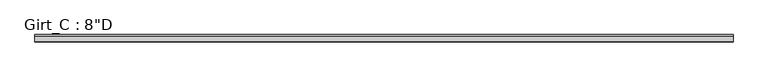
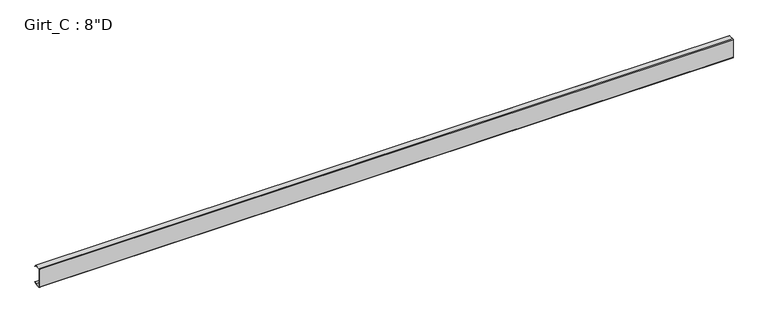
"""IFC4 building model written with IfcOpenShell, lengths in millimetres: beam geometry."""

import ifcopenshell
import ifcopenshell.guid

model = None  # the IFC model being written
_history = None  # IfcOwnerHistory: only IFC2X3 demands one
_inside = {}  # id of a spatial element -> (the spatial element, [elements in it])
_under = {}  # id of a project, library or spatial element -> (it, [spatial elements below it])
_declared = {}  # id of a project -> (the project, [libraries it declares])
_typed = {}  # id of a type object -> (the type object, [elements of that type])
_made_of = {}  # id of a material, layer set ... -> (it, [elements and type objects made of it])


def new_model(schema):
    """Start an empty IFC model of exactly this schema.

    Asked for "IFC4X3", IfcOpenShell would pick the latest addendum, in which some entities
    have other attributes; the version numbers below select the first issue.
    IFC2X3 requires an IfcOwnerHistory on every rooted entity: one is made here for all.
    """
    global model, _history
    if schema == "IFC4X3":
        model = ifcopenshell.file(schema_version=(4, 3, 0, 0))
    else:
        model = ifcopenshell.file(schema=schema)
    _inside.clear()
    _under.clear()
    _declared.clear()
    _typed.clear()
    _made_of.clear()
    _history = None
    if model.schema == "IFC2X3":
        org = make("IfcOrganization", Name="unknown")
        user = make(
            "IfcPersonAndOrganization",
            ThePerson=make("IfcPerson", FamilyName="unknown"),
            TheOrganization=org,
        )
        app = make(
            "IfcApplication",
            ApplicationDeveloper=org,
            Version="unknown",
            ApplicationFullName="unknown",
            ApplicationIdentifier="unknown",
        )
        _history = make(
            "IfcOwnerHistory",
            OwningUser=user,
            OwningApplication=app,
            ChangeAction="ADDED",
            CreationDate=0,
        )
    return model


def make(cls, **values):
    """One entity of the class cls with the attributes given. An attribute that is None is left unset."""
    return model.create_entity(
        cls, **{name: value for name, value in values.items() if value is not None}
    )


def rooted(cls, **values):
    """An entity with a GlobalId (a new one), such as an element, a storey or a relation."""
    return make(cls, GlobalId=ifcopenshell.guid.new(), OwnerHistory=_history, **values)


def si_unit(unit_type, name, prefix=None):
    """IfcSIUnit, for example si_unit("LENGTHUNIT", "METRE", prefix="MILLI")."""
    return make("IfcSIUnit", UnitType=unit_type, Prefix=prefix, Name=name)


def assignment(units):
    """IfcUnitAssignment: the units of a project."""
    return None if units is None else make("IfcUnitAssignment", Units=units)


def point(xyz):
    """IfcCartesianPoint."""
    return None if xyz is None else make("IfcCartesianPoint", Coordinates=xyz)


def direction(xyz):
    """IfcDirection."""
    return None if xyz is None else make("IfcDirection", DirectionRatios=xyz)


def frame(location, z_axis=None, x_axis=None):
    """IfcAxis2Placement3D, a coordinate frame: its origin and axes. An axis left out is left unset."""
    return make(
        "IfcAxis2Placement3D",
        Location=point(location),
        Axis=direction(z_axis),
        RefDirection=direction(x_axis),
    )


def frame_2d(location, x_axis=None):
    """IfcAxis2Placement2D, a coordinate frame in the plane: its origin and x axis."""
    return make(
        "IfcAxis2Placement2D", Location=point(location), RefDirection=direction(x_axis)
    )


def origin():
    """The frame at (0, 0, 0) with its axes left unset."""
    return frame((0.0, 0.0, 0.0))


def place(relative_to, where):
    """IfcLocalPlacement: puts the frame where relative to a parent placement (None: the world)."""
    return make(
        "IfcLocalPlacement", PlacementRelTo=relative_to, RelativePlacement=where
    )


def context(
    kind, dimensions, precision=None, world=None, true_north=None, identifier=None
):
    """IfcGeometricRepresentationContext, for example the 3D "Model" context."""
    return make(
        "IfcGeometricRepresentationContext",
        ContextIdentifier=identifier,
        ContextType=kind,
        CoordinateSpaceDimension=dimensions,
        Precision=precision,
        WorldCoordinateSystem=world,
        TrueNorth=true_north,
    )


def project(units=None, contexts=None):
    """IfcProject with its units and contexts."""
    return rooted(
        "IfcProject",
        Name="project",
        RepresentationContexts=contexts,
        UnitsInContext=assignment(units),
    )


def spatial(cls, under=None, at=None, **own):
    """A site, building, storey or space (cls), placed at a placement, below another one or the project."""
    s = rooted(cls, ObjectPlacement=at, **own)
    if under is not None:
        _under.setdefault(under.id(), (under, []))[1].append(s)
    return s


def polyline(points):
    """IfcPolyline through the points."""
    return make("IfcPolyline", Points=[point(p) for p in points])


def circle_curve(where, radius):
    """IfcCircle in the frame where."""
    return make("IfcCircle", Position=where, Radius=radius)


def trimmed(basis, trim1, trim2, sense, master):
    """IfcTrimmedCurve: the piece of a basis curve between two trims."""
    return make(
        "IfcTrimmedCurve",
        BasisCurve=basis,
        Trim1=trim1,
        Trim2=trim2,
        SenseAgreement=sense,
        MasterRepresentation=master,
    )


def segment(curve, same_sense, transition):
    """IfcCompositeCurveSegment."""
    return make(
        "IfcCompositeCurveSegment",
        Transition=transition,
        SameSense=same_sense,
        ParentCurve=curve,
    )


def composite_curve(segments, self_intersect=None):
    """IfcCompositeCurve: segments joined end to end."""
    return make("IfcCompositeCurve", Segments=segments, SelfIntersect=self_intersect)


def outline(outer, holes=None, kind="AREA"):
    """IfcArbitraryClosedProfileDef: a profile drawn as a closed curve; with holes, ...WithVoids."""
    if holes is None:
        return make("IfcArbitraryClosedProfileDef", ProfileType=kind, OuterCurve=outer)
    return make(
        "IfcArbitraryProfileDefWithVoids",
        ProfileType=kind,
        OuterCurve=outer,
        InnerCurves=holes,
    )


def extrude(swept, where, along, depth):
    """IfcExtrudedAreaSolid: the profile swept, set in the frame where, extruded along a direction by depth."""
    return make(
        "IfcExtrudedAreaSolid",
        SweptArea=swept,
        Position=where,
        ExtrudedDirection=direction(along),
        Depth=depth,
    )


def shape(context_of_items, identifier, shape_type, items):
    """IfcShapeRepresentation: the items that make up one representation, for example the "Body"."""
    return make(
        "IfcShapeRepresentation",
        ContextOfItems=context_of_items,
        RepresentationIdentifier=identifier,
        RepresentationType=shape_type,
        Items=items,
    )


def source(mapping_origin, context_of_items, identifier, shape_type, items):
    """IfcRepresentationMap: a shape defined once, which mapped items show again and again."""
    return make(
        "IfcRepresentationMap",
        MappingOrigin=mapping_origin,
        MappedRepresentation=shape(context_of_items, identifier, shape_type, items),
    )


def transform(
    local_origin,
    x_axis=None,
    y_axis=None,
    z_axis=None,
    scale=None,
    scale2=None,
    scale3=None,
    uniform=True,
):
    """IfcCartesianTransformationOperator3D, or its non-uniform kind. x_axis, y_axis, z_axis: its Axis1, 2, 3."""
    if uniform:
        return make(
            "IfcCartesianTransformationOperator3D",
            Axis1=direction(x_axis),
            Axis2=direction(y_axis),
            LocalOrigin=point(local_origin),
            Scale=scale,
            Axis3=direction(z_axis),
        )
    return make(
        "IfcCartesianTransformationOperator3DnonUniform",
        Axis1=direction(x_axis),
        Axis2=direction(y_axis),
        LocalOrigin=point(local_origin),
        Scale=scale,
        Axis3=direction(z_axis),
        Scale2=scale2,
        Scale3=scale3,
    )


def mapped(mapping_source, mapping_target):
    """IfcMappedItem: shows the shape of a source again, moved by a transform."""
    return make(
        "IfcMappedItem", MappingSource=mapping_source, MappingTarget=mapping_target
    )


def made_of(thing, what):
    """Note that an element or type object is made of a material, layer set ...; save() writes the relation."""
    if what is not None:
        _made_of.setdefault(what.id(), (what, []))[1].append(thing)
    return thing


def element(
    cls,
    number,
    at=None,
    inside=None,
    cuts=None,
    type_object=None,
    material=None,
    context=None,
    identifier="Body",
    shape_type=None,
    held_by="IfcProductDefinitionShape",
    body=None,
    shapes=None,
    **own,
):
    """One element of the class cls, such as IfcWall. Its Tag is "e" and its number.

    at: its placement. inside: the storey or other place that contains it. cuts: it is an
    opening in that element (IfcRelVoidsElement). A single representation is given by context,
    identifier, shape_type and body (its items); several are given by shapes. held_by: the class
    of the entity that holds the representations. save() writes the other relations.
    """
    e = rooted(cls, Tag="e%d" % number, ObjectPlacement=at, **own)
    if body is not None:
        shapes = [shape(context, identifier, shape_type, body)]
    if shapes is not None:
        e.Representation = make(held_by, Representations=shapes)
    if inside is not None:
        _inside.setdefault(inside.id(), (inside, []))[1].append(e)
    if cuts is not None:
        rooted(
            "IfcRelVoidsElement", RelatingBuildingElement=cuts, RelatedOpeningElement=e
        )
    if type_object is not None:
        _typed.setdefault(type_object.id(), (type_object, []))[1].append(e)
    return made_of(e, material)


def aggregate(whole, parts):
    """IfcRelAggregates: a whole, such as a stair, and the parts it consists of."""
    return rooted("IfcRelAggregates", RelatingObject=whole, RelatedObjects=parts)


def save(model, path):
    """Write the relations noted so far, then the file.

    IfcRelAggregates (storeys below a building ...), IfcRelContainedInSpatialStructure (elements
    in a storey), IfcRelDefinesByType, IfcRelAssociatesMaterial and IfcRelDeclares: one each for
    every whole, place, type object, material and project.
    """
    for whole, parts in _under.values():
        aggregate(whole, parts)
    for where, things in _inside.values():
        rooted(
            "IfcRelContainedInSpatialStructure",
            RelatedElements=things,
            RelatingStructure=where,
        )
    for kind, things in _typed.values():
        rooted("IfcRelDefinesByType", RelatedObjects=things, RelatingType=kind)
    for what, things in _made_of.values():
        rooted("IfcRelAssociatesMaterial", RelatedObjects=things, RelatingMaterial=what)
    for by, libraries in _declared.values():
        rooted("IfcRelDeclares", RelatingContext=by, RelatedDefinitions=libraries)
    model.write(path)


def beam_645dcc2e(model_context):
    return source(origin(), model_context, "Body", "SweptSolid", [
        extrude(outline(composite_curve([segment(polyline([(63.5, 101.6), (75.745104, 87.0068534), (73.6169367, 85.221109), (62.204539, 98.821875), (3.3005807, 98.821875)]), True, "CONTINUOUS"), segment(trimmed(circle_curve(frame_2d((3.3741066, 96.8381931)), 1.9850441), [point((3.3005807, 98.821875))], [point((1.3890625, 96.8381931))], True, "CARTESIAN"), True, "CONTINUOUS"), segment(polyline([(1.3890625, 96.8381931), (1.3890625, -96.8389339)]), True, "CONTINUOUS"), segment(trimmed(circle_curve(frame_2d((3.3748024, -96.8389339)), 1.9857399), [point((1.3890625, -96.8389339))], [point((3.2694106, -98.821875))], True, "CARTESIAN"), True, "CONTINUOUS"), segment(polyline([(3.2694106, -98.821875), (62.204539, -98.821875), (73.6169367, -85.221109), (75.745104, -87.0068534), (63.5, -101.6), (3.3734375, -101.6)]), True, "CONTINUOUS"), segment(trimmed(circle_curve(frame_2d((3.3734375, -96.8375)), 4.7625), [point((3.3734375, -101.6))], [point((-1.3890625, -96.8375))], False, "CARTESIAN"), True, "CONTINUOUS"), segment(polyline([(-1.3890625, -96.8375), (-1.3890625, 96.8375)]), True, "CONTINUOUS"), segment(trimmed(circle_curve(frame_2d((3.3734375, 96.8375)), 4.7625), [point((-1.3890625, 96.8375))], [point((3.3734375, 101.6))], False, "CARTESIAN"), True, "CONTINUOUS"), segment(polyline([(3.3734375, 101.6), (63.5, 101.6)]), True, "CONTINUOUS")], self_intersect=False)), frame((-3509.16875, 0.0, 0.0), z_axis=(1.0, 0.0, 0.0), x_axis=(0.0, 1.0, 0.0)), (0.0, 0.0, 1.0), 7159.625),
    ])


if __name__ == "__main__":
    model = new_model("IFC4")
    model_context = context("Model", 3, world=origin())
    ifc_project = project(units=[si_unit("LENGTHUNIT", "METRE", prefix="MILLI")], contexts=[model_context])
    site = spatial("IfcSite", under=ifc_project)
    building = spatial("IfcBuilding", under=site)
    placement = place(None, origin())
    beam_shape = beam_645dcc2e(model_context)
    element("IfcBeam", 1, ObjectType="Girt_C : 8\"D", at=placement, inside=building, context=model_context, shape_type="MappedRepresentation", body=[
        mapped(beam_shape, transform((0.0, 0.0, 0.0), x_axis=(1.0, 0.0, 0.0), y_axis=(0.0, 1.0, 0.0), z_axis=(0.0, 0.0, 1.0))),
    ])
    save(model, "model.ifc")

# Revit data of these elements
# Type "Girt_C : 8\"D"
#   Web_Thickness = 0' - 0 7/64"
#   Length [instance default] = 10' - 0"
#   Leg_1 = 0' - 2 1/2"
#   Height = 0' - 8"
#   Structural Material [instance default] = none
# Element 1 (IfcBeam, "Girt_C : 8\"D")
#   Structural Material = Steel
#   Materials on its faces: "Steel"
# Materials
#   "Steel": class "Metal", colour RGB 118 118 114, transparency 0, Description = "Steel, mill finish", Cost = 0
